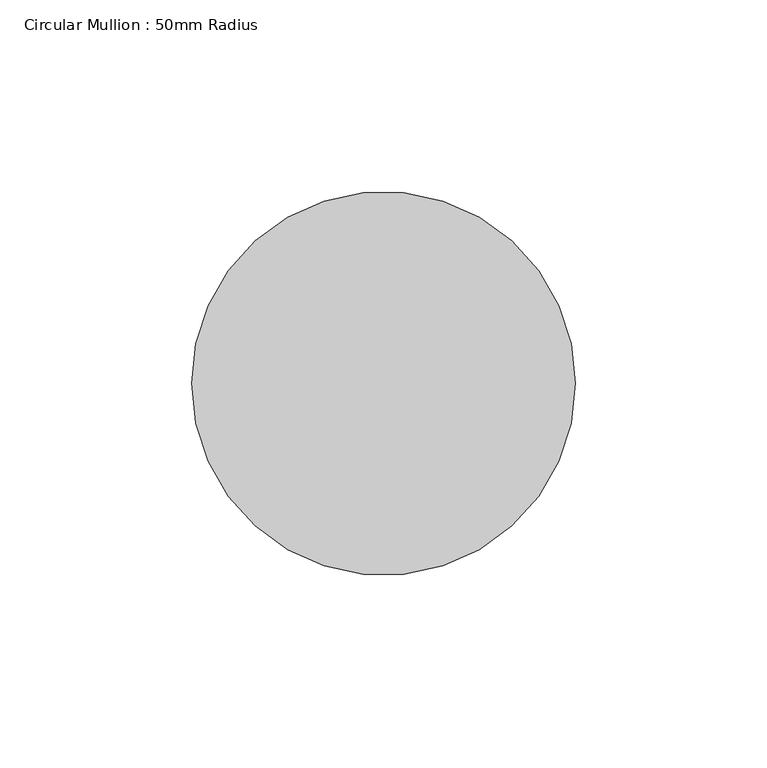
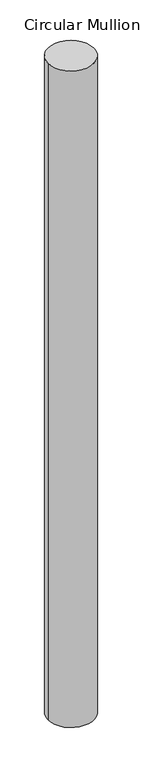
"""IFC4 building model written with IfcOpenShell, lengths in millimetres: member geometry, Circular Mullion : 50mm Radius."""

from ifc_helpers import new_model, si_unit, point, frame, origin, origin_2d, place, context, project, spatial, circle_curve, trimmed, segment, composite_curve, outline, extrude, source, transform, mapped, element, save


def circular_mullion_50mm_radius_cd29b567(model_context):
    return source(origin(), model_context, "Body", "SweptSolid", [
        extrude(outline(composite_curve([segment(trimmed(circle_curve(origin_2d(), 50.0), [point((50.0, 0.0))], [point((-50.0, 0.0))], False, "CARTESIAN"), True, "CONTINUOUS"), segment(trimmed(circle_curve(origin_2d(), 50.0), [point((-50.0, 0.0))], [point((50.0, 0.0))], False, "CARTESIAN"), True, "CONTINUOUS")], self_intersect=False)), frame((0.0, 0.0, -1510.7060193), z_axis=(0.0, 0.0, 1.0), x_axis=(1.0, 0.0, 0.0)), (0.0, 0.0, 1.0), 1510.7060193),
    ])


if __name__ == "__main__":
    model = new_model("IFC4")
    model_context = context("Model", 3, world=origin())
    ifc_project = project(units=[si_unit("LENGTHUNIT", "METRE", prefix="MILLI")], contexts=[model_context])
    site = spatial("IfcSite", under=ifc_project)
    building = spatial("IfcBuilding", under=site)
    placement = place(None, origin())
    circular_mullion_50mm_radius_shape = circular_mullion_50mm_radius_cd29b567(model_context)
    element("IfcMember", 1, ObjectType="Circular Mullion : 50mm Radius", at=placement, inside=building, context=model_context, shape_type="MappedRepresentation", body=[
        mapped(circular_mullion_50mm_radius_shape, transform((0.0, 0.0, 0.0), x_axis=(1.0, 0.0, 0.0), y_axis=(0.0, 1.0, 0.0), z_axis=(0.0, 0.0, 1.0))),
    ])
    save(model, "model.ifc")

# Revit data of these elements
# Type "Circular Mullion : 50mm Radius"
#   built-in parameter 1007350 = 0.164042 (stored number, unit not read)
# Element 1 (IfcMember, "Circular Mullion : 50mm Radius")
#   Materials on its faces: "Aluminium"
# Materials
#   "Aluminium": class "Metal", colour RGB 247 247 247, transparency 0, Description = "Aluminium 6061", Cost = 0
